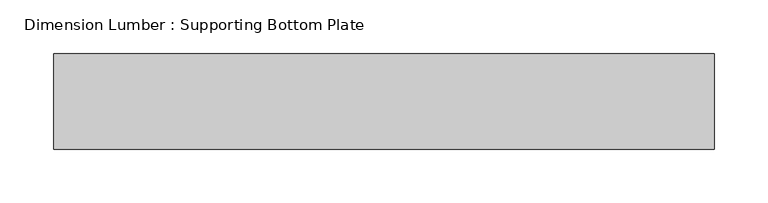
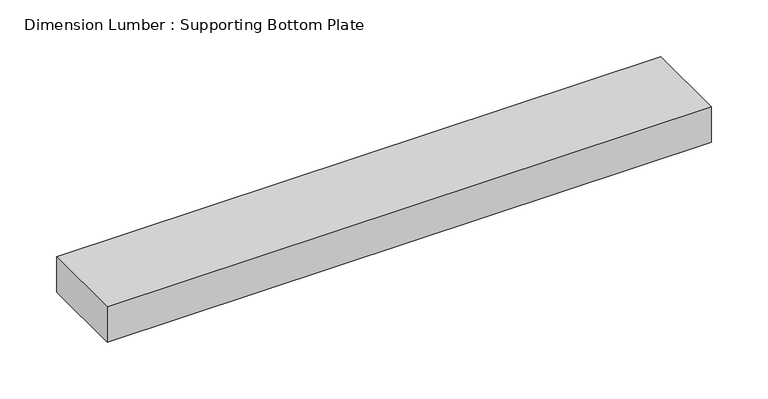
"""IFC4 building model written with IfcOpenShell, lengths in millimetres: beam geometry, Dimension Lumber : Supporting Bottom Plate."""

from ifc_helpers import new_model, si_unit, frame, origin, place, context, project, spatial, polyline, outline, extrude, source, transform, mapped, element, save


def dimension_lumber_supporting_bottom_plate_42822fc3(model_context):
    return source(origin(), model_context, "Body", "SweptSolid", [
        extrude(outline(polyline([(285.5562925, -44.45), (-330.0062925, -44.45), (-330.0062925, 44.45), (285.5562925, 44.45), (285.5562925, -44.45)])), frame((0.0, 0.0, -19.05), z_axis=(0.0, 0.0, 1.0), x_axis=(1.0, 0.0, 0.0)), (0.0, 0.0, 1.0), 38.1),
    ])


if __name__ == "__main__":
    model = new_model("IFC4")
    model_context = context("Model", 3, world=origin())
    ifc_project = project(units=[si_unit("LENGTHUNIT", "METRE", prefix="MILLI")], contexts=[model_context])
    site = spatial("IfcSite", under=ifc_project)
    building = spatial("IfcBuilding", under=site)
    placement = place(None, origin())
    dimension_lumber_supporting_bottom_plate_shape = dimension_lumber_supporting_bottom_plate_42822fc3(model_context)
    element("IfcBeam", 1, ObjectType="Dimension Lumber : Supporting Bottom Plate", at=placement, inside=building, context=model_context, shape_type="MappedRepresentation", body=[
        mapped(dimension_lumber_supporting_bottom_plate_shape, transform((0.0, 0.0, 0.0), x_axis=(1.0, 0.0, 0.0), y_axis=(0.0, 1.0, 0.0), z_axis=(0.0, 0.0, 1.0))),
    ])
    save(model, "model.ifc")

# Revit data of these elements
# Type "Dimension Lumber : Supporting Bottom Plate"
#   Assembly Code = "B10"
#   A = 0.0364583 SF
#   Length [instance default] = 5' - 0"
#   b = 0' - 3 1/2"
#   d = 0' - 1 1/2"
#   Structural Material [instance default] = Softwood, Lumber
# Element 1 (IfcBeam, "Dimension Lumber : Supporting Bottom Plate")
#   Structural Material = Douglas Fir #2
#   Materials on its faces: "Douglas Fir #2"
# Materials
#   "Softwood, Lumber": class "Wood", colour RGB 223 192 134, transparency 0, Description = "Pinus Echinata", Cost = 0
#   "Douglas Fir #2": class "Wood", colour RGB 223 192 134, transparency 0, Description = "Pinus Echinata", Cost = 0
